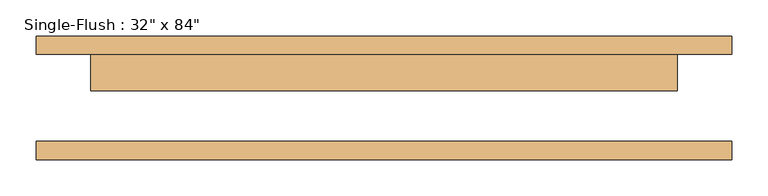
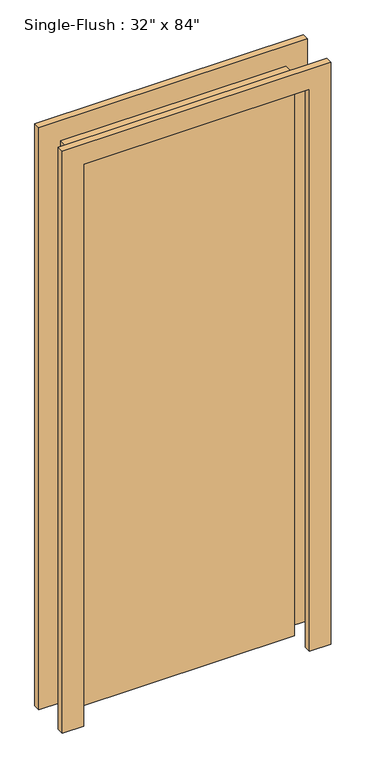
"""IFC4 building model written with IfcOpenShell, lengths in millimetres: door geometry."""

from ifc_helpers import new_model, si_unit, frame, origin, origin_with_axes, place, context, project, spatial, polyline, outline, extrude, source, transform, mapped, element, save


def door_5e27a1ea(model_context):
    return source(origin(), model_context, "Body", "SweptSolid", [
        extrude(outline(polyline([(2209.8, -482.6), (0.0, -482.6), (0.0, -406.4), (2133.6, -406.4), (2133.6, 406.4), (0.0, 406.4), (0.0, 482.6), (2209.8, 482.6), (2209.8, -482.6)])), frame((0.0, 60.325, 0.0), z_axis=(0.0, 1.0, 0.0), x_axis=(0.0, 0.0, 1.0)), (0.0, 0.0, 1.0), 25.4),
        extrude(outline(polyline([(2209.8, 482.6), (2209.8, -482.6), (0.0, -482.6), (0.0, -406.4), (2133.6, -406.4), (2133.6, 406.4), (0.0, 406.4), (0.0, 482.6), (2209.8, 482.6)])), frame((0.0, -85.725, 0.0), z_axis=(0.0, 1.0, 0.0), x_axis=(0.0, 0.0, 1.0)), (0.0, 0.0, 1.0), 25.4),
        extrude(outline(polyline([(406.4, 9.525), (-406.4, 9.525), (-406.4, 60.325), (406.4, 60.325), (406.4, 9.525)])), origin_with_axes(), (0.0, 0.0, 1.0), 2133.6),
    ])


if __name__ == "__main__":
    model = new_model("IFC4")
    model_context = context("Model", 3, world=origin())
    ifc_project = project(units=[si_unit("LENGTHUNIT", "METRE", prefix="MILLI")], contexts=[model_context])
    site = spatial("IfcSite", under=ifc_project)
    building = spatial("IfcBuilding", under=site)
    placement = place(None, origin())
    door_shape = door_5e27a1ea(model_context)
    element("IfcDoor", 1, ObjectType="Single-Flush : 32\" x 84\"", at=placement, inside=building, context=model_context, shape_type="MappedRepresentation", body=[
        mapped(door_shape, transform((0.0, 0.0, 0.0), x_axis=(1.0, 0.0, 0.0), y_axis=(0.0, 1.0, 0.0), z_axis=(0.0, 0.0, 1.0))),
    ])
    save(model, "model.ifc")

# Revit data of these elements
# Type "Single-Flush : 32\" x 84\""
#   Type Mark = "10"
#   Construction Type Id = "MDOOR"
#   Assembly Code = "C1020"
#   Analytic Construction = "Metal"
#   Thickness = 0' - 2"
#   Heat Transfer Coefficient (U) = 3.7021 W/(m²·K)
#   Height = 7' - 0"
#   Trim Projection Ext = 0' - 1"
#   Trim Projection Int = 0' - 1"
#   Trim Width = 0' - 3"
#   Width = 2' - 8"
#   Door Material = Door - Panel
#   Frame Material = Door - Frame
#   Visual Light Transmittance = 0
#   Solar Heat Gain Coefficient = 0
#   Function = (empty or 0)
#   Wall Closure = (empty or 0)
# Element 1 (IfcDoor, "Single-Flush : 32\" x 84\"")
#   Materials on its faces: "Door - Frame", "Door - Panel"
# Materials
#   "Door - Panel": class "Wood", colour RGB 210 159 95, transparency 0
#   "Door - Frame": class "Miscellaneous", colour RGB 118 70 51, transparency 0
